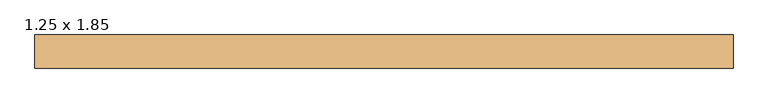
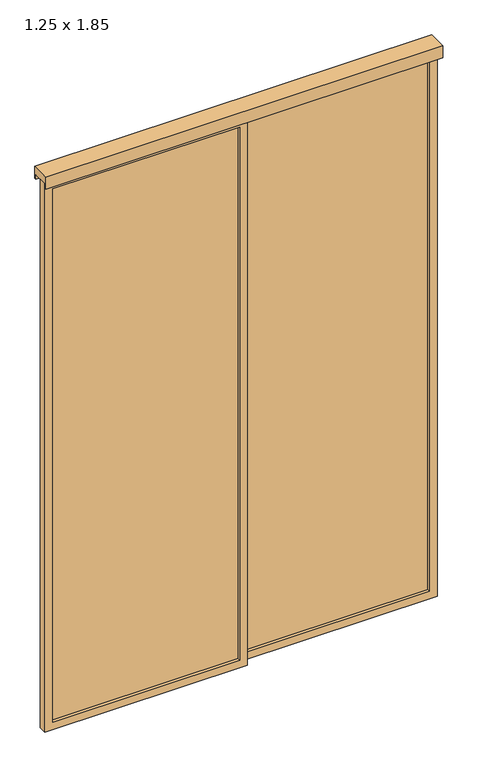
"""IFC4 building model written with IfcOpenShell, lengths in millimetres: door geometry, CC_ND-200_BOX-BANHEIRO : 1.25 x 1.85."""

from ifc_helpers import new_model, si_unit, frame, origin, place, context, project, spatial, polyline, outline, extrude, faceted_brep, source, transform, mapped, element, save


def door_1_25_x_1_85_04f1ac89(model_context):
    return source(origin(), model_context, "Body", "SolidModel", [
        extrude(outline(polyline([(627.5, 15.0), (627.5, 10.0), (10.0, 10.0), (10.0, 15.0), (627.5, 15.0)])), frame((0.0, 0.0, 10.0), z_axis=(0.0, 0.0, 1.0), x_axis=(1.0, 0.0, 0.0)), (0.0, 0.0, 1.0), 1805.0),
        faceted_brep([(612.5, 15.0, 1800.0), (612.5, 25.0, 1800.0), (612.5, 25.0, 25.0), (612.5, 15.0, 25.0), (637.5, 25.0, 1825.0), (637.5, 25.0, 0.0), (0.0, 25.0, 0.0), (0.0, 25.0, 1825.0), (25.0, 25.0, 1800.0), (25.0, 25.0, 25.0), (25.0, 15.0, 25.0), (10.0, 15.0, 1815.0), (10.0, 15.0, 10.0), (627.5, 15.0, 10.0), (627.5, 15.0, 1815.0), (25.0, 15.0, 1800.0), (637.5, 0.0, 1825.0), (637.5, 0.0, 0.0), (0.0, 0.0, 1825.0), (0.0, 0.0, 0.0), (612.5, 0.0, 1800.0), (612.5, 0.0, 25.0), (25.0, 0.0, 25.0), (25.0, 0.0, 1800.0), (612.5, 10.0, 1800.0), (612.5, 10.0, 25.0), (25.0, 10.0, 25.0), (25.0, 10.0, 1800.0), (627.5, 10.0, 1815.0), (627.5, 10.0, 10.0), (10.0, 10.0, 10.0), (10.0, 10.0, 1815.0)], [[[0, 1, 2, 3]], [[4, 5, 6, 7], [8, 9, 2, 1]], [[3, 2, 9, 10]], [[11, 12, 13, 14], [0, 3, 10, 15]], [[4, 16, 17, 5]], [[18, 19, 17, 16], [20, 21, 22, 23]], [[5, 17, 19, 6]], [[10, 9, 8, 15]], [[6, 19, 18, 7]], [[20, 24, 25, 21]], [[21, 25, 26, 22]], [[22, 26, 27, 23]], [[28, 14, 13, 29]], [[29, 13, 12, 30]], [[28, 29, 30, 31], [27, 26, 25, 24]], [[30, 12, 11, 31]], [[15, 8, 1, 0]], [[7, 18, 16, 4]], [[31, 11, 14, 28]], [[23, 27, 24, 20]]]),
        extrude(outline(polyline([(1240.0, 40.0), (1240.0, 35.0), (622.5, 35.0), (622.5, 40.0), (1240.0, 40.0)])), frame((0.0, 0.0, 10.0), z_axis=(0.0, 0.0, 1.0), x_axis=(1.0, 0.0, 0.0)), (0.0, 0.0, 1.0), 1805.0),
        faceted_brep([(1225.0, 40.0, 1800.0), (1225.0, 50.0, 1800.0), (1225.0, 50.0, 25.0), (1225.0, 40.0, 25.0), (1250.0, 50.0, 1825.0), (1250.0, 50.0, 0.0), (612.5, 50.0, 0.0), (612.5, 50.0, 1825.0), (637.5, 50.0, 1800.0), (637.5, 50.0, 25.0), (637.5, 40.0, 25.0), (622.5, 40.0, 1815.0), (622.5, 40.0, 10.0), (1240.0, 40.0, 10.0), (1240.0, 40.0, 1815.0), (637.5, 40.0, 1800.0), (1250.0, 25.0, 1825.0), (1250.0, 25.0, 0.0), (612.5, 25.0, 1825.0), (612.5, 25.0, 0.0), (1225.0, 25.0, 1800.0), (1225.0, 25.0, 25.0), (637.5, 25.0, 25.0), (637.5, 25.0, 1800.0), (1225.0, 35.0, 1800.0), (1225.0, 35.0, 25.0), (637.5, 35.0, 25.0), (637.5, 35.0, 1800.0), (1240.0, 35.0, 1815.0), (1240.0, 35.0, 10.0), (622.5, 35.0, 10.0), (622.5, 35.0, 1815.0)], [[[0, 1, 2, 3]], [[4, 5, 6, 7], [8, 9, 2, 1]], [[3, 2, 9, 10]], [[11, 12, 13, 14], [0, 3, 10, 15]], [[4, 16, 17, 5]], [[18, 19, 17, 16], [20, 21, 22, 23]], [[5, 17, 19, 6]], [[10, 9, 8, 15]], [[6, 19, 18, 7]], [[20, 24, 25, 21]], [[21, 25, 26, 22]], [[22, 26, 27, 23]], [[28, 14, 13, 29]], [[29, 13, 12, 30]], [[28, 29, 30, 31], [27, 26, 25, 24]], [[30, 12, 11, 31]], [[15, 8, 1, 0]], [[7, 18, 16, 4]], [[31, 11, 14, 28]], [[23, 27, 24, 20]]]),
        extrude(outline(polyline([(-5.0, 1810.0), (-5.0, 1850.0), (55.0, 1850.0), (55.0, 1810.0), (50.0, 1810.0), (50.0, 1825.0), (0.0, 1825.0), (0.0, 1810.0), (-5.0, 1810.0)])), frame((0.0, 0.0, 0.0), z_axis=(1.0, 0.0, 0.0), x_axis=(0.0, 1.0, 0.0)), (0.0, 0.0, 1.0), 1250.0),
    ])


if __name__ == "__main__":
    model = new_model("IFC4")
    model_context = context("Model", 3, world=origin())
    ifc_project = project(units=[si_unit("LENGTHUNIT", "METRE", prefix="MILLI")], contexts=[model_context])
    site = spatial("IfcSite", under=ifc_project)
    building = spatial("IfcBuilding", under=site)
    placement = place(None, origin())
    door_1_25_x_1_85_shape = door_1_25_x_1_85_04f1ac89(model_context)
    element("IfcDoor", 1, ObjectType="CC_ND-200_BOX-BANHEIRO : 1.25 x 1.85", at=placement, inside=building, context=model_context, shape_type="MappedRepresentation", body=[
        mapped(door_1_25_x_1_85_shape, transform((0.0, 0.0, 0.0), x_axis=(1.0, 0.0, 0.0), y_axis=(0.0, 1.0, 0.0), z_axis=(0.0, 0.0, 1.0))),
    ])
    save(model, "model.ifc")

# Revit data of these elements
# Type "CC_ND-200_BOX-BANHEIRO : 1.25 x 1.85"
#   Type Mark = "150"
#   Width = 1.25 m
#   Material montante = Aluminio
#   Materia vidro = Vidro
# Element 1 (IfcDoor, "CC_ND-200_BOX-BANHEIRO : 1.25 x 1.85")
#   Materials on its faces: "Aluminio", "Vidro"
# Materials
#   "Aluminio": class "Genérico", colour RGB 120 120 120, transparency 0, Cost = 0
#   "Vidro": class "Vidro", colour RGB 230 230 230, transparency 0.75, Description = "JANELA COM 04 FOLHAS DE CORRER E VIDRO TRANSPARENTE 6mm", Cost = 0
